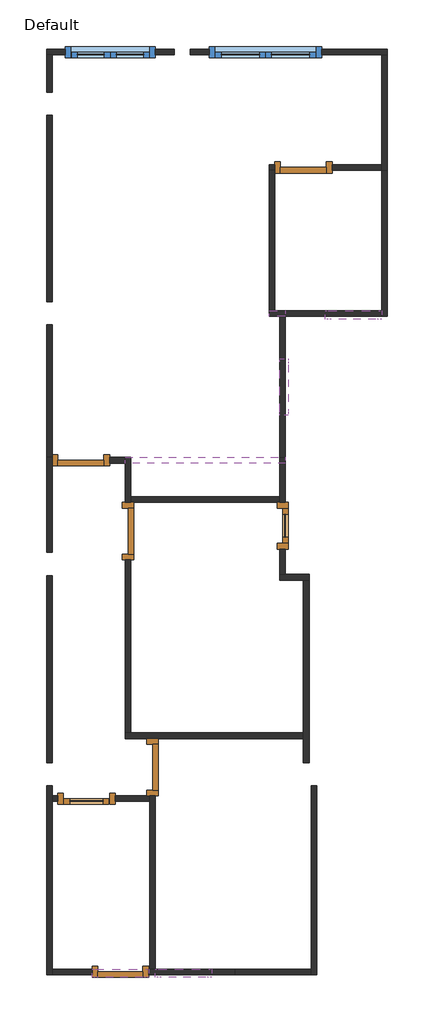
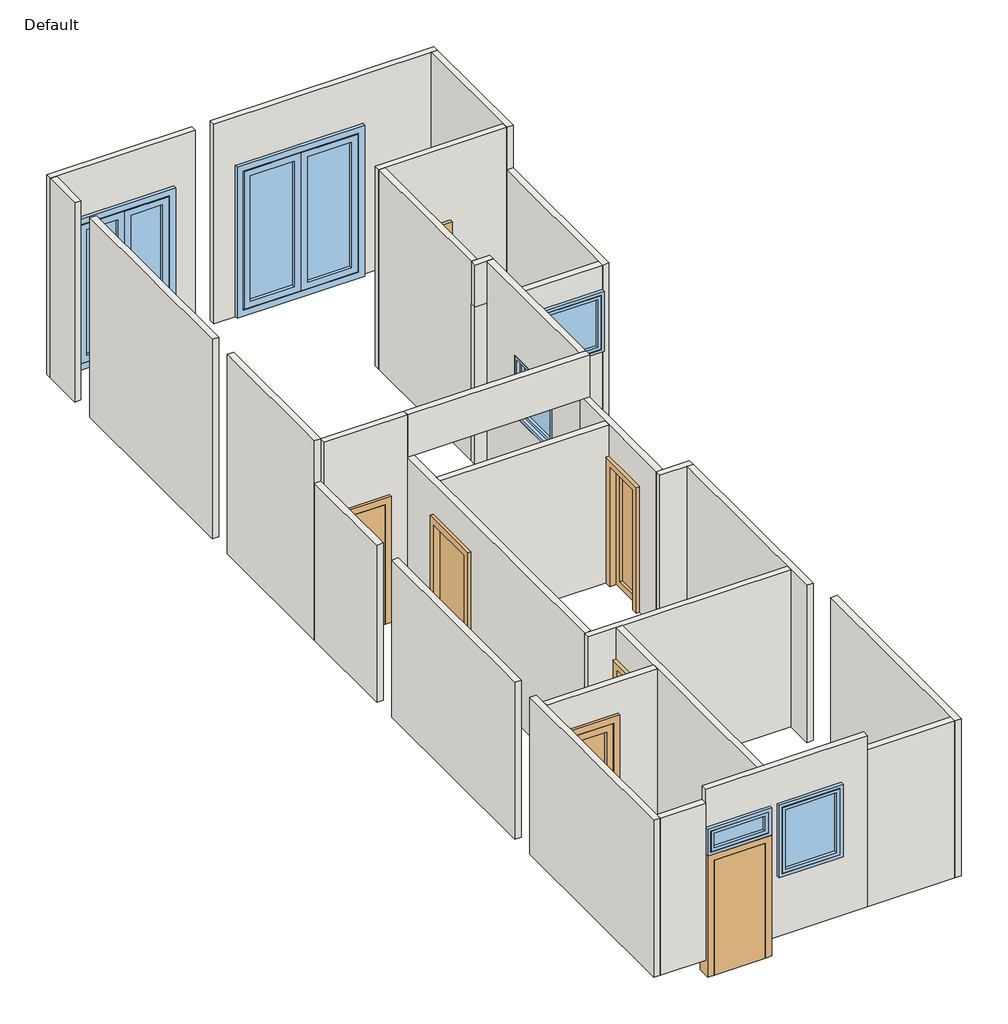
# One storey: 29 walls, 7 doors, 6 windows.
"""IFC4 building model written with IfcOpenShell, lengths in millimetres."""

import ifcopenshell
import ifcopenshell.guid

model = None  # the IFC model being written
_history = None  # IfcOwnerHistory: only IFC2X3 demands one
_inside = {}  # id of a spatial element -> (the spatial element, [elements in it])
_under = {}  # id of a project, library or spatial element -> (it, [spatial elements below it])
_declared = {}  # id of a project -> (the project, [libraries it declares])
_typed = {}  # id of a type object -> (the type object, [elements of that type])
_made_of = {}  # id of a material, layer set ... -> (it, [elements and type objects made of it])


def new_model(schema):
    """Start an empty IFC model of exactly this schema.

    Asked for "IFC4X3", IfcOpenShell would pick the latest addendum, in which some entities
    have other attributes; the version numbers below select the first issue.
    IFC2X3 requires an IfcOwnerHistory on every rooted entity: one is made here for all.
    """
    global model, _history
    if schema == "IFC4X3":
        model = ifcopenshell.file(schema_version=(4, 3, 0, 0))
    else:
        model = ifcopenshell.file(schema=schema)
    _inside.clear()
    _under.clear()
    _declared.clear()
    _typed.clear()
    _made_of.clear()
    _history = None
    if model.schema == "IFC2X3":
        org = make("IfcOrganization", Name="unknown")
        user = make(
            "IfcPersonAndOrganization",
            ThePerson=make("IfcPerson", FamilyName="unknown"),
            TheOrganization=org,
        )
        app = make(
            "IfcApplication",
            ApplicationDeveloper=org,
            Version="unknown",
            ApplicationFullName="unknown",
            ApplicationIdentifier="unknown",
        )
        _history = make(
            "IfcOwnerHistory",
            OwningUser=user,
            OwningApplication=app,
            ChangeAction="ADDED",
            CreationDate=0,
        )
    return model


def make(cls, **values):
    """One entity of the class cls with the attributes given. An attribute that is None is left unset."""
    return model.create_entity(
        cls, **{name: value for name, value in values.items() if value is not None}
    )


def rooted(cls, **values):
    """An entity with a GlobalId (a new one), such as an element, a storey or a relation."""
    return make(cls, GlobalId=ifcopenshell.guid.new(), OwnerHistory=_history, **values)


def si_unit(unit_type, name, prefix=None):
    """IfcSIUnit, for example si_unit("LENGTHUNIT", "METRE", prefix="MILLI")."""
    return make("IfcSIUnit", UnitType=unit_type, Prefix=prefix, Name=name)


def assignment(units):
    """IfcUnitAssignment: the units of a project."""
    return None if units is None else make("IfcUnitAssignment", Units=units)


def point(xyz):
    """IfcCartesianPoint."""
    return None if xyz is None else make("IfcCartesianPoint", Coordinates=xyz)


def direction(xyz):
    """IfcDirection."""
    return None if xyz is None else make("IfcDirection", DirectionRatios=xyz)


def frame(location, z_axis=None, x_axis=None):
    """IfcAxis2Placement3D, a coordinate frame: its origin and axes. An axis left out is left unset."""
    return make(
        "IfcAxis2Placement3D",
        Location=point(location),
        Axis=direction(z_axis),
        RefDirection=direction(x_axis),
    )


def origin():
    """The frame at (0, 0, 0) with its axes left unset."""
    return frame((0.0, 0.0, 0.0))


def origin_with_axes():
    """The frame at (0, 0, 0) with the z axis (0, 0, 1) and the x axis (1, 0, 0) written out."""
    return frame((0.0, 0.0, 0.0), z_axis=(0.0, 0.0, 1.0), x_axis=(1.0, 0.0, 0.0))


def place(relative_to, where):
    """IfcLocalPlacement: puts the frame where relative to a parent placement (None: the world)."""
    return make(
        "IfcLocalPlacement", PlacementRelTo=relative_to, RelativePlacement=where
    )


def context(
    kind, dimensions, precision=None, world=None, true_north=None, identifier=None
):
    """IfcGeometricRepresentationContext, for example the 3D "Model" context."""
    return make(
        "IfcGeometricRepresentationContext",
        ContextIdentifier=identifier,
        ContextType=kind,
        CoordinateSpaceDimension=dimensions,
        Precision=precision,
        WorldCoordinateSystem=world,
        TrueNorth=true_north,
    )


def project(units=None, contexts=None):
    """IfcProject with its units and contexts."""
    return rooted(
        "IfcProject",
        Name="project",
        RepresentationContexts=contexts,
        UnitsInContext=assignment(units),
    )


def spatial(cls, under=None, at=None, **own):
    """A site, building, storey or space (cls), placed at a placement, below another one or the project."""
    s = rooted(cls, ObjectPlacement=at, **own)
    if under is not None:
        _under.setdefault(under.id(), (under, []))[1].append(s)
    return s


def polyline(points):
    """IfcPolyline through the points."""
    return make("IfcPolyline", Points=[point(p) for p in points])


def outline(outer, holes=None, kind="AREA"):
    """IfcArbitraryClosedProfileDef: a profile drawn as a closed curve; with holes, ...WithVoids."""
    if holes is None:
        return make("IfcArbitraryClosedProfileDef", ProfileType=kind, OuterCurve=outer)
    return make(
        "IfcArbitraryProfileDefWithVoids",
        ProfileType=kind,
        OuterCurve=outer,
        InnerCurves=holes,
    )


def extrude(swept, where, along, depth):
    """IfcExtrudedAreaSolid: the profile swept, set in the frame where, extruded along a direction by depth."""
    return make(
        "IfcExtrudedAreaSolid",
        SweptArea=swept,
        Position=where,
        ExtrudedDirection=direction(along),
        Depth=depth,
    )


def shape(context_of_items, identifier, shape_type, items):
    """IfcShapeRepresentation: the items that make up one representation, for example the "Body"."""
    return make(
        "IfcShapeRepresentation",
        ContextOfItems=context_of_items,
        RepresentationIdentifier=identifier,
        RepresentationType=shape_type,
        Items=items,
    )


def source(mapping_origin, context_of_items, identifier, shape_type, items):
    """IfcRepresentationMap: a shape defined once, which mapped items show again and again."""
    return make(
        "IfcRepresentationMap",
        MappingOrigin=mapping_origin,
        MappedRepresentation=shape(context_of_items, identifier, shape_type, items),
    )


def transform(
    local_origin,
    x_axis=None,
    y_axis=None,
    z_axis=None,
    scale=None,
    scale2=None,
    scale3=None,
    uniform=True,
):
    """IfcCartesianTransformationOperator3D, or its non-uniform kind. x_axis, y_axis, z_axis: its Axis1, 2, 3."""
    if uniform:
        return make(
            "IfcCartesianTransformationOperator3D",
            Axis1=direction(x_axis),
            Axis2=direction(y_axis),
            LocalOrigin=point(local_origin),
            Scale=scale,
            Axis3=direction(z_axis),
        )
    return make(
        "IfcCartesianTransformationOperator3DnonUniform",
        Axis1=direction(x_axis),
        Axis2=direction(y_axis),
        LocalOrigin=point(local_origin),
        Scale=scale,
        Axis3=direction(z_axis),
        Scale2=scale2,
        Scale3=scale3,
    )


def mapped(mapping_source, mapping_target):
    """IfcMappedItem: shows the shape of a source again, moved by a transform."""
    return make(
        "IfcMappedItem", MappingSource=mapping_source, MappingTarget=mapping_target
    )


def made_of(thing, what):
    """Note that an element or type object is made of a material, layer set ...; save() writes the relation."""
    if what is not None:
        _made_of.setdefault(what.id(), (what, []))[1].append(thing)
    return thing


def element(
    cls,
    number,
    at=None,
    inside=None,
    cuts=None,
    type_object=None,
    material=None,
    context=None,
    identifier="Body",
    shape_type=None,
    held_by="IfcProductDefinitionShape",
    body=None,
    shapes=None,
    **own,
):
    """One element of the class cls, such as IfcWall. Its Tag is "e" and its number.

    at: its placement. inside: the storey or other place that contains it. cuts: it is an
    opening in that element (IfcRelVoidsElement). A single representation is given by context,
    identifier, shape_type and body (its items); several are given by shapes. held_by: the class
    of the entity that holds the representations. save() writes the other relations.
    """
    e = rooted(cls, Tag="e%d" % number, ObjectPlacement=at, **own)
    if body is not None:
        shapes = [shape(context, identifier, shape_type, body)]
    if shapes is not None:
        e.Representation = make(held_by, Representations=shapes)
    if inside is not None:
        _inside.setdefault(inside.id(), (inside, []))[1].append(e)
    if cuts is not None:
        rooted(
            "IfcRelVoidsElement", RelatingBuildingElement=cuts, RelatedOpeningElement=e
        )
    if type_object is not None:
        _typed.setdefault(type_object.id(), (type_object, []))[1].append(e)
    return made_of(e, material)


def aggregate(whole, parts):
    """IfcRelAggregates: a whole, such as a stair, and the parts it consists of."""
    return rooted("IfcRelAggregates", RelatingObject=whole, RelatedObjects=parts)


def save(model, path):
    """Write the relations noted so far, then the file.

    IfcRelAggregates (storeys below a building ...), IfcRelContainedInSpatialStructure (elements
    in a storey), IfcRelDefinesByType, IfcRelAssociatesMaterial and IfcRelDeclares: one each for
    every whole, place, type object, material and project.
    """
    for whole, parts in _under.values():
        aggregate(whole, parts)
    for where, things in _inside.values():
        rooted(
            "IfcRelContainedInSpatialStructure",
            RelatedElements=things,
            RelatingStructure=where,
        )
    for kind, things in _typed.values():
        rooted("IfcRelDefinesByType", RelatedObjects=things, RelatingType=kind)
    for what, things in _made_of.values():
        rooted("IfcRelAssociatesMaterial", RelatedObjects=things, RelatingMaterial=what)
    for by, libraries in _declared.values():
        rooted("IfcRelDeclares", RelatingContext=by, RelatedDefinitions=libraries)
    model.write(path)


def bathroom_door_bathroom_door_15b6a89a(model_context):
    return source(origin(), model_context, "Body", "SweptSolid", [
        extrude(outline(polyline([(4275.0, 14755.0), (5095.0, 14755.0), (5095.0, 14655.0), (4275.0, 14655.0), (4275.0, 14755.0)])), frame((0.0, 0.0, 250.0), z_axis=(0.0, 0.0, 1.0), x_axis=(1.0, 0.0, 0.0)), (0.0, 0.0, 1.0), 1980.0),
        extrude(outline(polyline([(250.0, 4175.0), (250.0, 4275.0), (2230.0, 4275.0), (2230.0, 5095.0), (250.0, 5095.0), (250.0, 5195.0), (2330.0, 5195.0), (2330.0, 4175.0), (250.0, 4175.0)])), frame((0.0, 14655.0, 0.0), z_axis=(0.0, 1.0, 0.0), x_axis=(0.0, 0.0, 1.0)), (0.0, 0.0, 1.0), 200.0),
    ])


def bedroom_1_door_bedroom_1_door_f4a16035(model_context):
    return source(origin(), model_context, "Body", "SweptSolid", [
        extrude(outline(polyline([(2000.0, 3675.0), (2000.0, 4495.0), (2100.0, 4495.0), (2100.0, 3675.0), (2000.0, 3675.0)])), frame((0.0, 0.0, 250.0), z_axis=(0.0, 0.0, 1.0), x_axis=(1.0, 0.0, 0.0)), (0.0, 0.0, 1.0), 1980.0),
        extrude(outline(polyline([(4595.0, 250.0), (4495.0, 250.0), (4495.0, 2230.0), (3675.0, 2230.0), (3675.0, 250.0), (3575.0, 250.0), (3575.0, 2330.0), (4595.0, 2330.0), (4595.0, 250.0)])), frame((1900.0, 0.0, 0.0), z_axis=(1.0, 0.0, 0.0), x_axis=(0.0, 1.0, 0.0)), (0.0, 0.0, 1.0), 200.0),
    ])


def bedroom_2_door_bedroom_2_door_3f2e3542(model_context):
    return source(origin(), model_context, "Body", "SweptSolid", [
        extrude(outline(polyline([(1565.0, 7875.0), (1565.0, 8695.0), (1665.0, 8695.0), (1665.0, 7875.0), (1565.0, 7875.0)])), frame((0.0, 0.0, 250.0), z_axis=(0.0, 0.0, 1.0), x_axis=(1.0, 0.0, 0.0)), (0.0, 0.0, 1.0), 1980.0),
        extrude(outline(polyline([(8795.0, 250.0), (8695.0, 250.0), (8695.0, 2230.0), (7875.0, 2230.0), (7875.0, 250.0), (7775.0, 250.0), (7775.0, 2330.0), (8795.0, 2330.0), (8795.0, 250.0)])), frame((1465.0, 0.0, 0.0), z_axis=(1.0, 0.0, 0.0), x_axis=(0.0, 1.0, 0.0)), (0.0, 0.0, 1.0), 200.0),
    ])


def bedroom_2_glass_door_bedroom_2_glass_door_faeb561c(model_context):
    return source(origin(), model_context, "Body", "SweptSolid", [
        extrude(outline(polyline([(4355.0, 8175.0), (4355.0, 8585.0), (4365.0, 8585.0), (4365.0, 8175.0), (4355.0, 8175.0)])), frame((0.0, 0.0, 360.0), z_axis=(0.0, 0.0, 1.0), x_axis=(1.0, 0.0, 0.0)), (0.0, 0.0, 1.0), 1760.0),
        extrude(outline(polyline([(8685.0, 2220.0), (8685.0, 260.0), (8075.0, 260.0), (8075.0, 2220.0), (8685.0, 2220.0)]), holes=[polyline([(8585.0, 360.0), (8585.0, 2120.0), (8175.0, 2120.0), (8175.0, 360.0), (8585.0, 360.0)])]), frame((4315.0, 0.0, 0.0), z_axis=(1.0, 0.0, 0.0), x_axis=(0.0, 1.0, 0.0)), (0.0, 0.0, 1.0), 100.0),
        extrude(outline(polyline([(8795.0, 250.0), (8695.0, 250.0), (8695.0, 2230.0), (8065.0, 2230.0), (8065.0, 250.0), (7965.0, 250.0), (7965.0, 2330.0), (8795.0, 2330.0), (8795.0, 250.0)])), frame((4215.0, 0.0, 0.0), z_axis=(1.0, 0.0, 0.0), x_axis=(0.0, 1.0, 0.0)), (0.0, 0.0, 1.0), 200.0),
    ])


def corridor_door_corridor_door_22811d5d(model_context):
    return source(origin(), model_context, "Body", "SweptSolid", [
        extrude(outline(polyline([(525.0, 3485.0), (1125.0, 3485.0), (1125.0, 3475.0), (525.0, 3475.0), (525.0, 3485.0)])), frame((0.0, 0.0, 360.0), z_axis=(0.0, 0.0, 1.0), x_axis=(1.0, 0.0, 0.0)), (0.0, 0.0, 1.0), 1760.0),
        extrude(outline(polyline([(260.0, 1225.0), (2220.0, 1225.0), (2220.0, 425.0), (260.0, 425.0), (260.0, 1225.0)]), holes=[polyline([(360.0, 525.0), (2120.0, 525.0), (2120.0, 1125.0), (360.0, 1125.0), (360.0, 525.0)])]), frame((0.0, 3425.0, 0.0), z_axis=(0.0, 1.0, 0.0), x_axis=(0.0, 0.0, 1.0)), (0.0, 0.0, 1.0), 100.0),
        extrude(outline(polyline([(250.0, 315.0), (250.0, 415.0), (2230.0, 415.0), (2230.0, 1235.0), (250.0, 1235.0), (250.0, 1335.0), (2330.0, 1335.0), (2330.0, 315.0), (250.0, 315.0)])), frame((0.0, 3425.0, 0.0), z_axis=(0.0, 1.0, 0.0), x_axis=(0.0, 0.0, 1.0)), (0.0, 0.0, 1.0), 200.0),
    ])


def front_door_front_door_f10339a7(model_context):
    return source(origin(), model_context, "Body", "SweptSolid", [
        extrude(outline(polyline([(1030.0, 445.0), (1830.0, 445.0), (1830.0, 345.0), (1030.0, 345.0), (1030.0, 445.0)])), origin_with_axes(), (0.0, 0.0, 1.0), 1900.0),
        extrude(outline(polyline([(0.0, 930.0), (0.0, 1030.0), (1900.0, 1030.0), (1900.0, 1830.0), (0.0, 1830.0), (0.0, 1930.0), (2000.0, 1930.0), (2000.0, 930.0), (0.0, 930.0)])), frame((0.0, 345.0, 0.0), z_axis=(0.0, 1.0, 0.0), x_axis=(0.0, 0.0, 1.0)), (0.0, 0.0, 1.0), 200.0),
    ])


def living_room_door_living_room_door_3c1abd9c(model_context):
    return source(origin(), model_context, "Body", "SweptSolid", [
        extrude(outline(polyline([(315.0, 9545.0), (1135.0, 9545.0), (1135.0, 9445.0), (315.0, 9445.0), (315.0, 9545.0)])), frame((0.0, 0.0, 250.0), z_axis=(0.0, 0.0, 1.0), x_axis=(1.0, 0.0, 0.0)), (0.0, 0.0, 1.0), 1980.0),
        extrude(outline(polyline([(250.0, 215.0), (250.0, 315.0), (2230.0, 315.0), (2230.0, 1135.0), (250.0, 1135.0), (250.0, 1235.0), (2330.0, 1235.0), (2330.0, 215.0), (250.0, 215.0)])), frame((0.0, 9445.0, 0.0), z_axis=(0.0, 1.0, 0.0), x_axis=(0.0, 0.0, 1.0)), (0.0, 0.0, 1.0), 200.0),
    ])


def steel_wall_1_steel_wall_1_b92ec2ca(model_context):
    return source(origin(), model_context, "Body", "SweptSolid", [
        extrude(outline(polyline([(215.0, 3755.0), (215.0, 395.0), (115.0, 395.0), (115.0, 3755.0), (215.0, 3755.0)])), frame((0.0, 0.0, 250.0), z_axis=(0.0, 0.0, 1.0), x_axis=(1.0, 0.0, 0.0)), (0.0, 0.0, 1.0), 2600.0),
    ])


def steel_wall_10_1_steel_wall_10_1_b84ba1d7(model_context):
    return source(origin(), model_context, "Body", "SweptSolid", [
        extrude(outline(polyline([(9595.0, 3550.0), (12105.0, 3550.0), (12105.0, 250.0), (9595.0, 250.0), (9595.0, 3550.0)]), holes=[polyline([(11350.0, 2450.0), (10350.0, 2450.0), (10350.0, 1450.0), (11350.0, 1450.0), (11350.0, 2450.0)])]), frame((4265.0, 0.0, 0.0), z_axis=(1.0, 0.0, 0.0), x_axis=(0.0, 1.0, 0.0)), (0.0, 0.0, 1.0), 100.0),
    ])


def steel_wall_10_2_steel_wall_10_2_ac5a625b(model_context):
    return source(origin(), model_context, "Body", "SweptSolid", [
        extrude(outline(polyline([(7515.0, 2850.0), (9595.0, 2850.0), (9595.0, 250.0), (8795.0, 250.0), (8795.0, 2330.0), (7965.0, 2330.0), (7965.0, 250.0), (7515.0, 250.0), (7515.0, 2850.0)])), frame((4265.0, 0.0, 0.0), z_axis=(1.0, 0.0, 0.0), x_axis=(0.0, 1.0, 0.0)), (0.0, 0.0, 1.0), 100.0),
    ])


def steel_wall_11_steel_wall_11_b2c771ff(model_context):
    return source(origin(), model_context, "Body", "SweptSolid", [
        extrude(outline(polyline([(4785.0, 7415.0), (4265.0, 7415.0), (4265.0, 7515.0), (4785.0, 7515.0), (4785.0, 7415.0)])), frame((0.0, 0.0, 250.0), z_axis=(0.0, 0.0, 1.0), x_axis=(1.0, 0.0, 0.0)), (0.0, 0.0, 1.0), 2600.0),
    ])


def steel_wall_12_steel_wall_12_e47ad89f(model_context):
    return source(origin(), model_context, "Body", "SweptSolid", [
        extrude(outline(polyline([(4785.0, 7415.0), (4785.0, 4165.0), (4685.0, 4165.0), (4685.0, 7415.0), (4785.0, 7415.0)])), frame((0.0, 0.0, 250.0), z_axis=(0.0, 0.0, 1.0), x_axis=(1.0, 0.0, 0.0)), (0.0, 0.0, 1.0), 2600.0),
    ])


def steel_wall_13_steel_wall_13_94e184f7(model_context):
    return source(origin(), model_context, "Body", "SweptSolid", [
        extrude(outline(polyline([(4925.0, 3755.0), (4925.0, 395.0), (4825.0, 395.0), (4825.0, 3755.0), (4925.0, 3755.0)])), frame((0.0, 0.0, 250.0), z_axis=(0.0, 0.0, 1.0), x_axis=(1.0, 0.0, 0.0)), (0.0, 0.0, 1.0), 2600.0),
    ])


def steel_wall_14_1_steel_wall_14_1_bad66547(model_context):
    return source(origin(), model_context, "Body", "SweptSolid", [
        extrude(outline(polyline([(930.0, 395.0), (215.0, 395.0), (215.0, 495.0), (930.0, 495.0), (930.0, 395.0)])), frame((0.0, 0.0, 250.0), z_axis=(0.0, 0.0, 1.0), x_axis=(1.0, 0.0, 0.0)), (0.0, 0.0, 1.0), 2600.0),
    ])


def steel_wall_14_2_steel_wall_14_2_555e5885(model_context):
    return source(origin(), model_context, "Body", "SweptSolid", [
        extrude(outline(polyline([(3080.0, 3460.0), (3080.0, 930.0), (2450.0, 930.0), (2450.0, 1930.0), (250.0, 1930.0), (250.0, 3460.0), (3080.0, 3460.0)]), holes=[polyline([(2450.0, 2050.0), (2450.0, 3050.0), (1250.0, 3050.0), (1250.0, 2050.0), (2450.0, 2050.0)])]), frame((0.0, 395.0, 0.0), z_axis=(0.0, 1.0, 0.0), x_axis=(0.0, 0.0, 1.0)), (0.0, 0.0, 1.0), 100.0),
    ])


def steel_wall_14_3_steel_wall_14_3_bb8a6b82(model_context):
    return source(origin(), model_context, "Body", "SweptSolid", [
        extrude(outline(polyline([(4825.0, 395.0), (3460.0, 395.0), (3460.0, 495.0), (4825.0, 495.0), (4825.0, 395.0)])), frame((0.0, 0.0, 250.0), z_axis=(0.0, 0.0, 1.0), x_axis=(1.0, 0.0, 0.0)), (0.0, 0.0, 1.0), 2600.0),
    ])


def steel_wall_2_steel_wall_2_9d9e34b6(model_context):
    return source(origin(), model_context, "Body", "SweptSolid", [
        extrude(outline(polyline([(215.0, 7495.0), (215.0, 4165.0), (115.0, 4165.0), (115.0, 7495.0), (215.0, 7495.0)])), frame((0.0, 0.0, 250.0), z_axis=(0.0, 0.0, 1.0), x_axis=(1.0, 0.0, 0.0)), (0.0, 0.0, 1.0), 2600.0),
    ])


def steel_wall_3_1_steel_wall_3_1_bd8174d4(model_context):
    return source(origin(), model_context, "Body", "SweptSolid", [
        extrude(outline(polyline([(215.0, 9595.0), (215.0, 7905.0), (115.0, 7905.0), (115.0, 9595.0), (215.0, 9595.0)])), frame((0.0, 0.0, 250.0), z_axis=(0.0, 0.0, 1.0), x_axis=(1.0, 0.0, 0.0)), (0.0, 0.0, 1.0), 2600.0),
    ])


def steel_wall_3_2_steel_wall_3_2_60cdce26(model_context):
    return source(origin(), model_context, "Body", "SweptSolid", [
        extrude(outline(polyline([(215.0, 11955.0), (215.0, 9595.0), (115.0, 9595.0), (115.0, 11955.0), (215.0, 11955.0)])), frame((0.0, 0.0, 250.0), z_axis=(0.0, 0.0, 1.0), x_axis=(1.0, 0.0, 0.0)), (0.0, 0.0, 1.0), 3300.0),
    ])


def steel_wall_4_steel_wall_4_2983a264(model_context):
    return source(origin(), model_context, "Body", "SweptSolid", [
        extrude(outline(polyline([(215.0, 15685.0), (215.0, 12365.0), (115.0, 12365.0), (115.0, 15685.0), (215.0, 15685.0)])), frame((0.0, 0.0, 250.0), z_axis=(0.0, 0.0, 1.0), x_axis=(1.0, 0.0, 0.0)), (0.0, 0.0, 1.0), 3300.0),
    ])


def steel_wall_5_steel_wall_5_69cba077(model_context):
    return source(origin(), model_context, "Body", "SweptSolid", [
        extrude(outline(polyline([(215.0, 16755.0), (215.0, 16095.0), (115.0, 16095.0), (115.0, 16755.0), (215.0, 16755.0)])), frame((0.0, 0.0, 250.0), z_axis=(0.0, 0.0, 1.0), x_axis=(1.0, 0.0, 0.0)), (0.0, 0.0, 1.0), 3300.0),
    ])


def steel_wall_6_steel_wall_6_a34f8d7e(model_context):
    return source(origin(), model_context, "Body", "SweptSolid", [
        extrude(outline(polyline([(3550.0, 2385.0), (3550.0, 115.0), (250.0, 115.0), (250.0, 450.0), (2750.0, 450.0), (2750.0, 2050.0), (250.0, 2050.0), (250.0, 2385.0), (3550.0, 2385.0)])), frame((0.0, 16755.0, 0.0), z_axis=(0.0, 1.0, 0.0), x_axis=(0.0, 0.0, 1.0)), (0.0, 0.0, 1.0), 100.0),
    ])


def steel_wall_7_steel_wall_7_8661bafb(model_context):
    return source(origin(), model_context, "Body", "SweptSolid", [
        extrude(outline(polyline([(3550.0, 6175.0), (3550.0, 2675.0), (250.0, 2675.0), (250.0, 3010.0), (2750.0, 3010.0), (2750.0, 5010.0), (250.0, 5010.0), (250.0, 6175.0), (3550.0, 6175.0)])), frame((0.0, 16755.0, 0.0), z_axis=(0.0, 1.0, 0.0), x_axis=(0.0, 0.0, 1.0)), (0.0, 0.0, 1.0), 100.0),
    ])


def steel_wall_8_1_steel_wall_8_1_6002a07f(model_context):
    return source(origin(), model_context, "Body", "SweptSolid", [
        extrude(outline(polyline([(6175.0, 16755.0), (6175.0, 14705.0), (6075.0, 14705.0), (6075.0, 16755.0), (6175.0, 16755.0)])), frame((0.0, 0.0, 250.0), z_axis=(0.0, 0.0, 1.0), x_axis=(1.0, 0.0, 0.0)), (0.0, 0.0, 1.0), 3300.0),
    ])


def steel_wall_8_2_steel_wall_8_2_e95248a5(model_context):
    return source(origin(), model_context, "Body", "SweptSolid", [
        extrude(outline(polyline([(6175.0, 14705.0), (6175.0, 12105.0), (6075.0, 12105.0), (6075.0, 14705.0), (6175.0, 14705.0)])), frame((0.0, 0.0, 250.0), z_axis=(0.0, 0.0, 1.0), x_axis=(1.0, 0.0, 0.0)), (0.0, 0.0, 1.0), 2600.0),
    ])


def steel_wall_9_steel_wall_9_7bb1e214(model_context):
    return source(origin(), model_context, "Body", "SweptSolid", [
        extrude(outline(polyline([(2850.0, 6075.0), (2850.0, 4075.0), (250.0, 4075.0), (250.0, 6075.0), (1450.0, 6075.0), (1450.0, 5075.0), (2450.0, 5075.0), (2450.0, 6075.0), (2850.0, 6075.0)])), frame((0.0, 12105.0, 0.0), z_axis=(0.0, 1.0, 0.0), x_axis=(0.0, 0.0, 1.0)), (0.0, 0.0, 1.0), 100.0),
    ])


def steel_wall_bath_1_steel_wall_bath_1_50d80b11(model_context):
    return source(origin(), model_context, "Body", "SweptSolid", [
        extrude(outline(polyline([(4175.0, 14705.0), (4175.0, 12205.0), (4075.0, 12205.0), (4075.0, 14705.0), (4175.0, 14705.0)])), frame((0.0, 0.0, 250.0), z_axis=(0.0, 0.0, 1.0), x_axis=(1.0, 0.0, 0.0)), (0.0, 0.0, 1.0), 3300.0),
    ])


def steel_wall_bath_2_steel_wall_bath_2_118e7a6d(model_context):
    return source(origin(), model_context, "Body", "SweptSolid", [
        extrude(outline(polyline([(3550.0, 6075.0), (3550.0, 4075.0), (250.0, 4075.0), (250.0, 4175.0), (2330.0, 4175.0), (2330.0, 5195.0), (250.0, 5195.0), (250.0, 6075.0), (3550.0, 6075.0)])), frame((0.0, 14705.0, 0.0), z_axis=(0.0, 1.0, 0.0), x_axis=(0.0, 0.0, 1.0)), (0.0, 0.0, 1.0), 100.0),
    ])


def steel_wall_bath_3_steel_wall_bath_3_592d521f(model_context):
    return source(origin(), model_context, "Body", "SweptSolid", [
        extrude(outline(polyline([(4365.0, 12105.0), (4075.0, 12105.0), (4075.0, 12205.0), (4365.0, 12205.0), (4365.0, 12105.0)])), frame((0.0, 0.0, 2850.0), z_axis=(0.0, 0.0, 1.0), x_axis=(1.0, 0.0, 0.0)), (0.0, 0.0, 1.0), 700.0),
    ])


def steel_wall_bed_1_1_steel_wall_bed_1_1_07c56df4(model_context):
    return source(origin(), model_context, "Body", "SweptSolid", [
        extrude(outline(polyline([(495.0, 2850.0), (4595.0, 2850.0), (4595.0, 2330.0), (3575.0, 2330.0), (3575.0, 250.0), (495.0, 250.0), (495.0, 2850.0)])), frame((1950.0, 0.0, 0.0), z_axis=(1.0, 0.0, 0.0), x_axis=(0.0, 1.0, 0.0)), (0.0, 0.0, 1.0), 100.0),
    ])


def steel_wall_bed_1_2_steel_wall_bed_1_2_5afbed24(model_context):
    return source(origin(), model_context, "Body", "SweptSolid", [
        extrude(outline(polyline([(4685.0, 4595.0), (1515.0, 4595.0), (1515.0, 4695.0), (4685.0, 4695.0), (4685.0, 4595.0)])), frame((0.0, 0.0, 250.0), z_axis=(0.0, 0.0, 1.0), x_axis=(1.0, 0.0, 0.0)), (0.0, 0.0, 1.0), 2600.0),
    ])


def steel_wall_bed_2_1_steel_wall_bed_2_1_f0eb02fb(model_context):
    return source(origin(), model_context, "Body", "SweptSolid", [
        extrude(outline(polyline([(4695.0, 2850.0), (9595.0, 2850.0), (9595.0, 250.0), (8795.0, 250.0), (8795.0, 2330.0), (7775.0, 2330.0), (7775.0, 250.0), (4695.0, 250.0), (4695.0, 2850.0)])), frame((1515.0, 0.0, 0.0), z_axis=(1.0, 0.0, 0.0), x_axis=(0.0, 1.0, 0.0)), (0.0, 0.0, 1.0), 100.0),
    ])


def steel_wall_bed_2_2_steel_wall_bed_2_2_f5710ee6(model_context):
    return source(origin(), model_context, "Body", "SweptSolid", [
        extrude(outline(polyline([(4265.0, 8795.0), (1615.0, 8795.0), (1615.0, 8895.0), (4265.0, 8895.0), (4265.0, 8795.0)])), frame((0.0, 0.0, 250.0), z_axis=(0.0, 0.0, 1.0), x_axis=(1.0, 0.0, 0.0)), (0.0, 0.0, 1.0), 2600.0),
    ])


def steel_wall_corridor_1_steel_wall_corridor_1_64942479(model_context):
    return source(origin(), model_context, "Body", "SweptSolid", [
        extrude(outline(polyline([(2850.0, 1950.0), (2850.0, 215.0), (250.0, 215.0), (250.0, 315.0), (2330.0, 315.0), (2330.0, 1335.0), (250.0, 1335.0), (250.0, 1950.0), (2850.0, 1950.0)])), frame((0.0, 3475.0, 0.0), z_axis=(0.0, 1.0, 0.0), x_axis=(0.0, 0.0, 1.0)), (0.0, 0.0, 1.0), 100.0),
    ])


def steel_wall_corridor_2_steel_wall_corridor_2_3c3fb1a4(model_context):
    return source(origin(), model_context, "Body", "SweptSolid", [
        extrude(outline(polyline([(3550.0, 1515.0), (3550.0, 215.0), (2330.0, 215.0), (2330.0, 1235.0), (250.0, 1235.0), (250.0, 1515.0), (3550.0, 1515.0)])), frame((0.0, 9495.0, 0.0), z_axis=(0.0, 1.0, 0.0), x_axis=(0.0, 0.0, 1.0)), (0.0, 0.0, 1.0), 100.0),
    ])


def steel_wall_kitchen_steel_wall_kitchen_7f8e7296(model_context):
    return source(origin(), model_context, "Body", "SweptSolid", [
        extrude(outline(polyline([(4365.0, 9495.0), (1515.0, 9495.0), (1515.0, 9595.0), (4365.0, 9595.0), (4365.0, 9495.0)])), frame((0.0, 0.0, 2850.0), z_axis=(0.0, 0.0, 1.0), x_axis=(1.0, 0.0, 0.0)), (0.0, 0.0, 1.0), 700.0),
    ])


def bedroom_1_window_bedroom_1_window_a7b937d5(model_context):
    return source(origin(), model_context, "Body", "SweptSolid", [
        extrude(outline(polyline([(5180.0, 12115.0), (5970.0, 12115.0), (5970.0, 12105.0), (5180.0, 12105.0), (5180.0, 12115.0)])), frame((0.0, 0.0, 1555.0), z_axis=(0.0, 0.0, 1.0), x_axis=(1.0, 0.0, 0.0)), (0.0, 0.0, 1.0), 790.0),
        extrude(outline(polyline([(1505.0, 6020.0), (2395.0, 6020.0), (2395.0, 5130.0), (1505.0, 5130.0), (1505.0, 6020.0)]), holes=[polyline([(1555.0, 5180.0), (2345.0, 5180.0), (2345.0, 5970.0), (1555.0, 5970.0), (1555.0, 5180.0)])]), frame((0.0, 12055.0, 0.0), z_axis=(0.0, 1.0, 0.0), x_axis=(0.0, 0.0, 1.0)), (0.0, 0.0, 1.0), 100.0),
        extrude(outline(polyline([(1450.0, 6075.0), (2450.0, 6075.0), (2450.0, 5075.0), (1450.0, 5075.0), (1450.0, 6075.0)]), holes=[polyline([(1500.0, 5125.0), (2400.0, 5125.0), (2400.0, 6025.0), (1500.0, 6025.0), (1500.0, 5125.0)])]), frame((0.0, 12055.0, 0.0), z_axis=(0.0, 1.0, 0.0), x_axis=(0.0, 0.0, 1.0)), (0.0, 0.0, 1.0), 150.0),
    ])


def bedroom_1_window001_bedroom_1_window001_719b1152(model_context):
    return source(origin(), model_context, "Body", "SweptSolid", [
        extrude(outline(polyline([(2155.0, 405.0), (2945.0, 405.0), (2945.0, 395.0), (2155.0, 395.0), (2155.0, 405.0)])), frame((0.0, 0.0, 1355.0), z_axis=(0.0, 0.0, 1.0), x_axis=(1.0, 0.0, 0.0)), (0.0, 0.0, 1.0), 990.0),
        extrude(outline(polyline([(1305.0, 2995.0), (2395.0, 2995.0), (2395.0, 2105.0), (1305.0, 2105.0), (1305.0, 2995.0)]), holes=[polyline([(1355.0, 2155.0), (2345.0, 2155.0), (2345.0, 2945.0), (1355.0, 2945.0), (1355.0, 2155.0)])]), frame((0.0, 345.0, 0.0), z_axis=(0.0, 1.0, 0.0), x_axis=(0.0, 0.0, 1.0)), (0.0, 0.0, 1.0), 100.0),
        extrude(outline(polyline([(1250.0, 3050.0), (2450.0, 3050.0), (2450.0, 2050.0), (1250.0, 2050.0), (1250.0, 3050.0)]), holes=[polyline([(1300.0, 2100.0), (2400.0, 2100.0), (2400.0, 3000.0), (1300.0, 3000.0), (1300.0, 2100.0)])]), frame((0.0, 345.0, 0.0), z_axis=(0.0, 1.0, 0.0), x_axis=(0.0, 0.0, 1.0)), (0.0, 0.0, 1.0), 150.0),
    ])


def corridor_window_corridor_window_b9059d84(model_context):
    return source(origin(), model_context, "Body", "SweptSolid", [
        extrude(outline(polyline([(1035.0, 405.0), (1825.0, 405.0), (1825.0, 395.0), (1035.0, 395.0), (1035.0, 405.0)])), frame((0.0, 0.0, 2105.0), z_axis=(0.0, 0.0, 1.0), x_axis=(1.0, 0.0, 0.0)), (0.0, 0.0, 1.0), 240.0),
        extrude(outline(polyline([(2055.0, 1875.0), (2395.0, 1875.0), (2395.0, 985.0), (2055.0, 985.0), (2055.0, 1875.0)]), holes=[polyline([(2105.0, 1035.0), (2345.0, 1035.0), (2345.0, 1825.0), (2105.0, 1825.0), (2105.0, 1035.0)])]), frame((0.0, 345.0, 0.0), z_axis=(0.0, 1.0, 0.0), x_axis=(0.0, 0.0, 1.0)), (0.0, 0.0, 1.0), 100.0),
        extrude(outline(polyline([(2000.0, 1930.0), (2450.0, 1930.0), (2450.0, 930.0), (2000.0, 930.0), (2000.0, 1930.0)]), holes=[polyline([(2050.0, 980.0), (2400.0, 980.0), (2400.0, 1880.0), (2050.0, 1880.0), (2050.0, 980.0)])]), frame((0.0, 345.0, 0.0), z_axis=(0.0, 1.0, 0.0), x_axis=(0.0, 0.0, 1.0)), (0.0, 0.0, 1.0), 150.0),
    ])


def garden_door_1_garden_door_1_5a744e37(model_context):
    return source(origin(), model_context, "Body", "SweptSolid", [
        extrude(outline(polyline([(1355.0, 16765.0), (1840.0, 16765.0), (1840.0, 16755.0), (1355.0, 16755.0), (1355.0, 16765.0)])), frame((0.0, 0.0, 460.0), z_axis=(0.0, 0.0, 1.0), x_axis=(1.0, 0.0, 0.0)), (0.0, 0.0, 1.0), 2080.0),
        extrude(outline(polyline([(360.0, 1940.0), (2640.0, 1940.0), (2640.0, 1255.0), (360.0, 1255.0), (360.0, 1940.0)]), holes=[polyline([(460.0, 1355.0), (2540.0, 1355.0), (2540.0, 1840.0), (460.0, 1840.0), (460.0, 1355.0)])]), frame((0.0, 16705.0, 0.0), z_axis=(0.0, 1.0, 0.0), x_axis=(0.0, 0.0, 1.0)), (0.0, 0.0, 1.0), 100.0),
        extrude(outline(polyline([(660.0, 16765.0), (1145.0, 16765.0), (1145.0, 16755.0), (660.0, 16755.0), (660.0, 16765.0)])), frame((0.0, 0.0, 460.0), z_axis=(0.0, 0.0, 1.0), x_axis=(1.0, 0.0, 0.0)), (0.0, 0.0, 1.0), 2080.0),
        extrude(outline(polyline([(360.0, 1245.0), (2640.0, 1245.0), (2640.0, 560.0), (360.0, 560.0), (360.0, 1245.0)]), holes=[polyline([(460.0, 660.0), (2540.0, 660.0), (2540.0, 1145.0), (460.0, 1145.0), (460.0, 660.0)])]), frame((0.0, 16705.0, 0.0), z_axis=(0.0, 1.0, 0.0), x_axis=(0.0, 0.0, 1.0)), (0.0, 0.0, 1.0), 100.0),
        extrude(outline(polyline([(250.0, 2050.0), (2750.0, 2050.0), (2750.0, 450.0), (250.0, 450.0), (250.0, 2050.0)]), holes=[polyline([(350.0, 550.0), (2650.0, 550.0), (2650.0, 1950.0), (350.0, 1950.0), (350.0, 550.0)])]), frame((0.0, 16705.0, 0.0), z_axis=(0.0, 1.0, 0.0), x_axis=(0.0, 0.0, 1.0)), (0.0, 0.0, 1.0), 200.0),
    ])


def garden_door_2_garden_door_2_d5e40104(model_context):
    return source(origin(), model_context, "Body", "SweptSolid", [
        extrude(outline(polyline([(4115.0, 16765.0), (4800.0, 16765.0), (4800.0, 16755.0), (4115.0, 16755.0), (4115.0, 16765.0)])), frame((0.0, 0.0, 460.0), z_axis=(0.0, 0.0, 1.0), x_axis=(1.0, 0.0, 0.0)), (0.0, 0.0, 1.0), 2080.0),
        extrude(outline(polyline([(360.0, 4900.0), (2640.0, 4900.0), (2640.0, 4015.0), (360.0, 4015.0), (360.0, 4900.0)]), holes=[polyline([(460.0, 4115.0), (2540.0, 4115.0), (2540.0, 4800.0), (460.0, 4800.0), (460.0, 4115.0)])]), frame((0.0, 16705.0, 0.0), z_axis=(0.0, 1.0, 0.0), x_axis=(0.0, 0.0, 1.0)), (0.0, 0.0, 1.0), 100.0),
        extrude(outline(polyline([(3220.0, 16765.0), (3905.0, 16765.0), (3905.0, 16755.0), (3220.0, 16755.0), (3220.0, 16765.0)])), frame((0.0, 0.0, 460.0), z_axis=(0.0, 0.0, 1.0), x_axis=(1.0, 0.0, 0.0)), (0.0, 0.0, 1.0), 2080.0),
        extrude(outline(polyline([(360.0, 4005.0), (2640.0, 4005.0), (2640.0, 3120.0), (360.0, 3120.0), (360.0, 4005.0)]), holes=[polyline([(460.0, 3220.0), (2540.0, 3220.0), (2540.0, 3905.0), (460.0, 3905.0), (460.0, 3220.0)])]), frame((0.0, 16705.0, 0.0), z_axis=(0.0, 1.0, 0.0), x_axis=(0.0, 0.0, 1.0)), (0.0, 0.0, 1.0), 100.0),
        extrude(outline(polyline([(250.0, 5010.0), (2750.0, 5010.0), (2750.0, 3010.0), (250.0, 3010.0), (250.0, 5010.0)]), holes=[polyline([(350.0, 3110.0), (2650.0, 3110.0), (2650.0, 4910.0), (350.0, 4910.0), (350.0, 3110.0)])]), frame((0.0, 16705.0, 0.0), z_axis=(0.0, 1.0, 0.0), x_axis=(0.0, 0.0, 1.0)), (0.0, 0.0, 1.0), 200.0),
    ])


def kitchen_window_kitchen_window_f07ff302(model_context):
    return source(origin(), model_context, "Body", "SweptSolid", [
        extrude(outline(polyline([(4355.0, 10455.0), (4355.0, 11245.0), (4365.0, 11245.0), (4365.0, 10455.0), (4355.0, 10455.0)])), frame((0.0, 0.0, 1555.0), z_axis=(0.0, 0.0, 1.0), x_axis=(1.0, 0.0, 0.0)), (0.0, 0.0, 1.0), 790.0),
        extrude(outline(polyline([(11295.0, 2395.0), (11295.0, 1505.0), (10405.0, 1505.0), (10405.0, 2395.0), (11295.0, 2395.0)]), holes=[polyline([(11245.0, 1555.0), (11245.0, 2345.0), (10455.0, 2345.0), (10455.0, 1555.0), (11245.0, 1555.0)])]), frame((4315.0, 0.0, 0.0), z_axis=(1.0, 0.0, 0.0), x_axis=(0.0, 1.0, 0.0)), (0.0, 0.0, 1.0), 100.0),
        extrude(outline(polyline([(11350.0, 2450.0), (11350.0, 1450.0), (10350.0, 1450.0), (10350.0, 2450.0), (11350.0, 2450.0)]), holes=[polyline([(11300.0, 1500.0), (11300.0, 2400.0), (10400.0, 2400.0), (10400.0, 1500.0), (11300.0, 1500.0)])]), frame((4265.0, 0.0, 0.0), z_axis=(1.0, 0.0, 0.0), x_axis=(0.0, 1.0, 0.0)), (0.0, 0.0, 1.0), 150.0),
    ])


model = new_model("IFC4")

# Units and contexts
model_context = context("Model", 3, world=origin())
ifc_project = project(units=[si_unit("LENGTHUNIT", "METRE", prefix="MILLI")], contexts=[model_context])

# Site, building, storey
site = spatial("IfcSite", under=ifc_project)
building = spatial("IfcBuilding", under=site)
storey = spatial("IfcBuildingStorey", under=building, Name="Default", Elevation=0.0)

# Doors
placement = place(None, origin())
bathroom_door_bathroom_door_shape = bathroom_door_bathroom_door_15b6a89a(model_context)
element("IfcDoor", 1, ObjectType="Bathroom_Door : Bathroom_Door", at=placement, inside=storey, context=model_context, shape_type="MappedRepresentation", body=[
    mapped(bathroom_door_bathroom_door_shape, transform((0.0, 0.0, 0.0), x_axis=(1.0, 0.0, 0.0), y_axis=(0.0, 1.0, 0.0), z_axis=(0.0, 0.0, 1.0))),
])
bedroom_1_door_bedroom_1_door_shape = bedroom_1_door_bedroom_1_door_f4a16035(model_context)
element("IfcDoor", 2, ObjectType="Bedroom_1_Door : Bedroom_1_Door", at=placement, inside=storey, context=model_context, shape_type="MappedRepresentation", body=[
    mapped(bedroom_1_door_bedroom_1_door_shape, transform((0.0, 0.0, 0.0), x_axis=(1.0, 0.0, 0.0), y_axis=(0.0, 1.0, 0.0), z_axis=(0.0, 0.0, 1.0))),
])
bedroom_2_door_bedroom_2_door_shape = bedroom_2_door_bedroom_2_door_3f2e3542(model_context)
element("IfcDoor", 3, ObjectType="Bedroom_2_Door : Bedroom_2_Door", at=placement, inside=storey, context=model_context, shape_type="MappedRepresentation", body=[
    mapped(bedroom_2_door_bedroom_2_door_shape, transform((0.0, 0.0, 0.0), x_axis=(1.0, 0.0, 0.0), y_axis=(0.0, 1.0, 0.0), z_axis=(0.0, 0.0, 1.0))),
])
bedroom_2_glass_door_bedroom_2_glass_door_shape = bedroom_2_glass_door_bedroom_2_glass_door_faeb561c(model_context)
element("IfcDoor", 4, ObjectType="Bedroom_2__Glass_Door : Bedroom_2__Glass_Door", at=placement, inside=storey, context=model_context, shape_type="MappedRepresentation", body=[
    mapped(bedroom_2_glass_door_bedroom_2_glass_door_shape, transform((0.0, 0.0, 0.0), x_axis=(1.0, 0.0, 0.0), y_axis=(0.0, 1.0, 0.0), z_axis=(0.0, 0.0, 1.0))),
])
corridor_door_corridor_door_shape = corridor_door_corridor_door_22811d5d(model_context)
element("IfcDoor", 5, ObjectType="Corridor_Door : Corridor_Door", at=placement, inside=storey, context=model_context, shape_type="MappedRepresentation", body=[
    mapped(corridor_door_corridor_door_shape, transform((0.0, 0.0, 0.0), x_axis=(1.0, 0.0, 0.0), y_axis=(0.0, 1.0, 0.0), z_axis=(0.0, 0.0, 1.0))),
])
front_door_front_door_shape = front_door_front_door_f10339a7(model_context)
element("IfcDoor", 6, ObjectType="Front_Door : Front_Door", at=placement, inside=storey, context=model_context, shape_type="MappedRepresentation", body=[
    mapped(front_door_front_door_shape, transform((0.0, 0.0, 0.0), x_axis=(1.0, 0.0, 0.0), y_axis=(0.0, 1.0, 0.0), z_axis=(0.0, 0.0, 1.0))),
])
living_room_door_living_room_door_shape = living_room_door_living_room_door_3c1abd9c(model_context)
element("IfcDoor", 7, ObjectType="Living_Room_Door : Living_Room_Door", at=placement, inside=storey, context=model_context, shape_type="MappedRepresentation", body=[
    mapped(living_room_door_living_room_door_shape, transform((0.0, 0.0, 0.0), x_axis=(1.0, 0.0, 0.0), y_axis=(0.0, 1.0, 0.0), z_axis=(0.0, 0.0, 1.0))),
])

# Walls
steel_wall_1_steel_wall_1_shape = steel_wall_1_steel_wall_1_b92ec2ca(model_context)
element("IfcWall", 8, ObjectType="Steel_Wall_1 : Steel_Wall_1", at=placement, inside=storey, context=model_context, shape_type="MappedRepresentation", body=[
    mapped(steel_wall_1_steel_wall_1_shape, transform((0.0, 0.0, 0.0), x_axis=(1.0, 0.0, 0.0), y_axis=(0.0, 1.0, 0.0), z_axis=(0.0, 0.0, 1.0))),
])
steel_wall_10_1_steel_wall_10_1_shape = steel_wall_10_1_steel_wall_10_1_b84ba1d7(model_context)
element("IfcWall", 9, ObjectType="Steel_Wall_10_1 : Steel_Wall_10_1", at=placement, inside=storey, context=model_context, shape_type="MappedRepresentation", body=[
    mapped(steel_wall_10_1_steel_wall_10_1_shape, transform((0.0, 0.0, 0.0), x_axis=(1.0, 0.0, 0.0), y_axis=(0.0, 1.0, 0.0), z_axis=(0.0, 0.0, 1.0))),
])
steel_wall_10_2_steel_wall_10_2_shape = steel_wall_10_2_steel_wall_10_2_ac5a625b(model_context)
element("IfcWall", 10, ObjectType="Steel_Wall_10_2 : Steel_Wall_10_2", at=placement, inside=storey, context=model_context, shape_type="MappedRepresentation", body=[
    mapped(steel_wall_10_2_steel_wall_10_2_shape, transform((0.0, 0.0, 0.0), x_axis=(1.0, 0.0, 0.0), y_axis=(0.0, 1.0, 0.0), z_axis=(0.0, 0.0, 1.0))),
])
steel_wall_11_steel_wall_11_shape = steel_wall_11_steel_wall_11_b2c771ff(model_context)
element("IfcWall", 11, ObjectType="Steel_Wall_11 : Steel_Wall_11", at=placement, inside=storey, context=model_context, shape_type="MappedRepresentation", body=[
    mapped(steel_wall_11_steel_wall_11_shape, transform((0.0, 0.0, 0.0), x_axis=(1.0, 0.0, 0.0), y_axis=(0.0, 1.0, 0.0), z_axis=(0.0, 0.0, 1.0))),
])
steel_wall_12_steel_wall_12_shape = steel_wall_12_steel_wall_12_e47ad89f(model_context)
element("IfcWall", 12, ObjectType="Steel_Wall_12 : Steel_Wall_12", at=placement, inside=storey, context=model_context, shape_type="MappedRepresentation", body=[
    mapped(steel_wall_12_steel_wall_12_shape, transform((0.0, 0.0, 0.0), x_axis=(1.0, 0.0, 0.0), y_axis=(0.0, 1.0, 0.0), z_axis=(0.0, 0.0, 1.0))),
])
steel_wall_13_steel_wall_13_shape = steel_wall_13_steel_wall_13_94e184f7(model_context)
element("IfcWall", 13, ObjectType="Steel_Wall_13 : Steel_Wall_13", at=placement, inside=storey, context=model_context, shape_type="MappedRepresentation", body=[
    mapped(steel_wall_13_steel_wall_13_shape, transform((0.0, 0.0, 0.0), x_axis=(1.0, 0.0, 0.0), y_axis=(0.0, 1.0, 0.0), z_axis=(0.0, 0.0, 1.0))),
])
steel_wall_14_1_steel_wall_14_1_shape = steel_wall_14_1_steel_wall_14_1_bad66547(model_context)
element("IfcWall", 14, ObjectType="Steel_Wall_14_1 : Steel_Wall_14_1", at=placement, inside=storey, context=model_context, shape_type="MappedRepresentation", body=[
    mapped(steel_wall_14_1_steel_wall_14_1_shape, transform((0.0, 0.0, 0.0), x_axis=(1.0, 0.0, 0.0), y_axis=(0.0, 1.0, 0.0), z_axis=(0.0, 0.0, 1.0))),
])
steel_wall_14_2_steel_wall_14_2_shape = steel_wall_14_2_steel_wall_14_2_555e5885(model_context)
element("IfcWall", 15, ObjectType="Steel_Wall_14_2 : Steel_Wall_14_2", at=placement, inside=storey, context=model_context, shape_type="MappedRepresentation", body=[
    mapped(steel_wall_14_2_steel_wall_14_2_shape, transform((0.0, 0.0, 0.0), x_axis=(1.0, 0.0, 0.0), y_axis=(0.0, 1.0, 0.0), z_axis=(0.0, 0.0, 1.0))),
])
steel_wall_14_3_steel_wall_14_3_shape = steel_wall_14_3_steel_wall_14_3_bb8a6b82(model_context)
element("IfcWall", 16, ObjectType="Steel_Wall_14_3 : Steel_Wall_14_3", at=placement, inside=storey, context=model_context, shape_type="MappedRepresentation", body=[
    mapped(steel_wall_14_3_steel_wall_14_3_shape, transform((0.0, 0.0, 0.0), x_axis=(1.0, 0.0, 0.0), y_axis=(0.0, 1.0, 0.0), z_axis=(0.0, 0.0, 1.0))),
])
steel_wall_2_steel_wall_2_shape = steel_wall_2_steel_wall_2_9d9e34b6(model_context)
element("IfcWall", 17, ObjectType="Steel_Wall_2 : Steel_Wall_2", at=placement, inside=storey, context=model_context, shape_type="MappedRepresentation", body=[
    mapped(steel_wall_2_steel_wall_2_shape, transform((0.0, 0.0, 0.0), x_axis=(1.0, 0.0, 0.0), y_axis=(0.0, 1.0, 0.0), z_axis=(0.0, 0.0, 1.0))),
])
steel_wall_3_1_steel_wall_3_1_shape = steel_wall_3_1_steel_wall_3_1_bd8174d4(model_context)
element("IfcWall", 18, ObjectType="Steel_Wall_3_1 : Steel_Wall_3_1", at=placement, inside=storey, context=model_context, shape_type="MappedRepresentation", body=[
    mapped(steel_wall_3_1_steel_wall_3_1_shape, transform((0.0, 0.0, 0.0), x_axis=(1.0, 0.0, 0.0), y_axis=(0.0, 1.0, 0.0), z_axis=(0.0, 0.0, 1.0))),
])
steel_wall_3_2_steel_wall_3_2_shape = steel_wall_3_2_steel_wall_3_2_60cdce26(model_context)
element("IfcWall", 19, ObjectType="Steel_Wall_3_2 : Steel_Wall_3_2", at=placement, inside=storey, context=model_context, shape_type="MappedRepresentation", body=[
    mapped(steel_wall_3_2_steel_wall_3_2_shape, transform((0.0, 0.0, 0.0), x_axis=(1.0, 0.0, 0.0), y_axis=(0.0, 1.0, 0.0), z_axis=(0.0, 0.0, 1.0))),
])
steel_wall_4_steel_wall_4_shape = steel_wall_4_steel_wall_4_2983a264(model_context)
element("IfcWall", 20, ObjectType="Steel_Wall_4 : Steel_Wall_4", at=placement, inside=storey, context=model_context, shape_type="MappedRepresentation", body=[
    mapped(steel_wall_4_steel_wall_4_shape, transform((0.0, 0.0, 0.0), x_axis=(1.0, 0.0, 0.0), y_axis=(0.0, 1.0, 0.0), z_axis=(0.0, 0.0, 1.0))),
])
steel_wall_5_steel_wall_5_shape = steel_wall_5_steel_wall_5_69cba077(model_context)
element("IfcWall", 21, ObjectType="Steel_Wall_5 : Steel_Wall_5", at=placement, inside=storey, context=model_context, shape_type="MappedRepresentation", body=[
    mapped(steel_wall_5_steel_wall_5_shape, transform((0.0, 0.0, 0.0), x_axis=(1.0, 0.0, 0.0), y_axis=(0.0, 1.0, 0.0), z_axis=(0.0, 0.0, 1.0))),
])
steel_wall_6_steel_wall_6_shape = steel_wall_6_steel_wall_6_a34f8d7e(model_context)
element("IfcWall", 22, ObjectType="Steel_Wall_6 : Steel_Wall_6", at=placement, inside=storey, context=model_context, shape_type="MappedRepresentation", body=[
    mapped(steel_wall_6_steel_wall_6_shape, transform((0.0, 0.0, 0.0), x_axis=(1.0, 0.0, 0.0), y_axis=(0.0, 1.0, 0.0), z_axis=(0.0, 0.0, 1.0))),
])
steel_wall_7_steel_wall_7_shape = steel_wall_7_steel_wall_7_8661bafb(model_context)
element("IfcWall", 23, ObjectType="Steel_Wall_7 : Steel_Wall_7", at=placement, inside=storey, context=model_context, shape_type="MappedRepresentation", body=[
    mapped(steel_wall_7_steel_wall_7_shape, transform((0.0, 0.0, 0.0), x_axis=(1.0, 0.0, 0.0), y_axis=(0.0, 1.0, 0.0), z_axis=(0.0, 0.0, 1.0))),
])
steel_wall_8_1_steel_wall_8_1_shape = steel_wall_8_1_steel_wall_8_1_6002a07f(model_context)
element("IfcWall", 24, ObjectType="Steel_Wall_8_1 : Steel_Wall_8_1", at=placement, inside=storey, context=model_context, shape_type="MappedRepresentation", body=[
    mapped(steel_wall_8_1_steel_wall_8_1_shape, transform((0.0, 0.0, 0.0), x_axis=(1.0, 0.0, 0.0), y_axis=(0.0, 1.0, 0.0), z_axis=(0.0, 0.0, 1.0))),
])
steel_wall_8_2_steel_wall_8_2_shape = steel_wall_8_2_steel_wall_8_2_e95248a5(model_context)
element("IfcWall", 25, ObjectType="Steel_Wall_8_2 : Steel_Wall_8_2", at=placement, inside=storey, context=model_context, shape_type="MappedRepresentation", body=[
    mapped(steel_wall_8_2_steel_wall_8_2_shape, transform((0.0, 0.0, 0.0), x_axis=(1.0, 0.0, 0.0), y_axis=(0.0, 1.0, 0.0), z_axis=(0.0, 0.0, 1.0))),
])
steel_wall_9_steel_wall_9_shape = steel_wall_9_steel_wall_9_7bb1e214(model_context)
element("IfcWall", 26, ObjectType="Steel_Wall_9 : Steel_Wall_9", at=placement, inside=storey, context=model_context, shape_type="MappedRepresentation", body=[
    mapped(steel_wall_9_steel_wall_9_shape, transform((0.0, 0.0, 0.0), x_axis=(1.0, 0.0, 0.0), y_axis=(0.0, 1.0, 0.0), z_axis=(0.0, 0.0, 1.0))),
])
steel_wall_bath_1_steel_wall_bath_1_shape = steel_wall_bath_1_steel_wall_bath_1_50d80b11(model_context)
element("IfcWall", 27, ObjectType="Steel_Wall_Bath_1 : Steel_Wall_Bath_1", at=placement, inside=storey, context=model_context, shape_type="MappedRepresentation", body=[
    mapped(steel_wall_bath_1_steel_wall_bath_1_shape, transform((0.0, 0.0, 0.0), x_axis=(1.0, 0.0, 0.0), y_axis=(0.0, 1.0, 0.0), z_axis=(0.0, 0.0, 1.0))),
])
steel_wall_bath_2_steel_wall_bath_2_shape = steel_wall_bath_2_steel_wall_bath_2_118e7a6d(model_context)
element("IfcWall", 28, ObjectType="Steel_Wall_Bath_2 : Steel_Wall_Bath_2", at=placement, inside=storey, context=model_context, shape_type="MappedRepresentation", body=[
    mapped(steel_wall_bath_2_steel_wall_bath_2_shape, transform((0.0, 0.0, 0.0), x_axis=(1.0, 0.0, 0.0), y_axis=(0.0, 1.0, 0.0), z_axis=(0.0, 0.0, 1.0))),
])
steel_wall_bath_3_steel_wall_bath_3_shape = steel_wall_bath_3_steel_wall_bath_3_592d521f(model_context)
element("IfcWall", 29, ObjectType="Steel_Wall_Bath_3 : Steel_Wall_Bath_3", at=placement, inside=storey, context=model_context, shape_type="MappedRepresentation", body=[
    mapped(steel_wall_bath_3_steel_wall_bath_3_shape, transform((0.0, 0.0, 0.0), x_axis=(1.0, 0.0, 0.0), y_axis=(0.0, 1.0, 0.0), z_axis=(0.0, 0.0, 1.0))),
])
steel_wall_bed_1_1_steel_wall_bed_1_1_shape = steel_wall_bed_1_1_steel_wall_bed_1_1_07c56df4(model_context)
element("IfcWall", 30, ObjectType="Steel_Wall_Bed_1_1 : Steel_Wall_Bed_1_1", at=placement, inside=storey, context=model_context, shape_type="MappedRepresentation", body=[
    mapped(steel_wall_bed_1_1_steel_wall_bed_1_1_shape, transform((0.0, 0.0, 0.0), x_axis=(1.0, 0.0, 0.0), y_axis=(0.0, 1.0, 0.0), z_axis=(0.0, 0.0, 1.0))),
])
steel_wall_bed_1_2_steel_wall_bed_1_2_shape = steel_wall_bed_1_2_steel_wall_bed_1_2_5afbed24(model_context)
element("IfcWall", 31, ObjectType="Steel_Wall_Bed_1_2 : Steel_Wall_Bed_1_2", at=placement, inside=storey, context=model_context, shape_type="MappedRepresentation", body=[
    mapped(steel_wall_bed_1_2_steel_wall_bed_1_2_shape, transform((0.0, 0.0, 0.0), x_axis=(1.0, 0.0, 0.0), y_axis=(0.0, 1.0, 0.0), z_axis=(0.0, 0.0, 1.0))),
])
steel_wall_bed_2_1_steel_wall_bed_2_1_shape = steel_wall_bed_2_1_steel_wall_bed_2_1_f0eb02fb(model_context)
element("IfcWall", 32, ObjectType="Steel_Wall_Bed_2_1 : Steel_Wall_Bed_2_1", at=placement, inside=storey, context=model_context, shape_type="MappedRepresentation", body=[
    mapped(steel_wall_bed_2_1_steel_wall_bed_2_1_shape, transform((0.0, 0.0, 0.0), x_axis=(1.0, 0.0, 0.0), y_axis=(0.0, 1.0, 0.0), z_axis=(0.0, 0.0, 1.0))),
])
steel_wall_bed_2_2_steel_wall_bed_2_2_shape = steel_wall_bed_2_2_steel_wall_bed_2_2_f5710ee6(model_context)
element("IfcWall", 33, ObjectType="Steel_Wall_Bed_2_2 : Steel_Wall_Bed_2_2", at=placement, inside=storey, context=model_context, shape_type="MappedRepresentation", body=[
    mapped(steel_wall_bed_2_2_steel_wall_bed_2_2_shape, transform((0.0, 0.0, 0.0), x_axis=(1.0, 0.0, 0.0), y_axis=(0.0, 1.0, 0.0), z_axis=(0.0, 0.0, 1.0))),
])
steel_wall_corridor_1_steel_wall_corridor_1_shape = steel_wall_corridor_1_steel_wall_corridor_1_64942479(model_context)
element("IfcWall", 34, ObjectType="Steel_Wall_Corridor_1 : Steel_Wall_Corridor_1", at=placement, inside=storey, context=model_context, shape_type="MappedRepresentation", body=[
    mapped(steel_wall_corridor_1_steel_wall_corridor_1_shape, transform((0.0, 0.0, 0.0), x_axis=(1.0, 0.0, 0.0), y_axis=(0.0, 1.0, 0.0), z_axis=(0.0, 0.0, 1.0))),
])
steel_wall_corridor_2_steel_wall_corridor_2_shape = steel_wall_corridor_2_steel_wall_corridor_2_3c3fb1a4(model_context)
element("IfcWall", 35, ObjectType="Steel_Wall_Corridor_2 : Steel_Wall_Corridor_2", at=placement, inside=storey, context=model_context, shape_type="MappedRepresentation", body=[
    mapped(steel_wall_corridor_2_steel_wall_corridor_2_shape, transform((0.0, 0.0, 0.0), x_axis=(1.0, 0.0, 0.0), y_axis=(0.0, 1.0, 0.0), z_axis=(0.0, 0.0, 1.0))),
])
steel_wall_kitchen_steel_wall_kitchen_shape = steel_wall_kitchen_steel_wall_kitchen_7f8e7296(model_context)
element("IfcWall", 36, ObjectType="Steel_Wall_Kitchen : Steel_Wall_Kitchen", at=placement, inside=storey, context=model_context, shape_type="MappedRepresentation", body=[
    mapped(steel_wall_kitchen_steel_wall_kitchen_shape, transform((0.0, 0.0, 0.0), x_axis=(1.0, 0.0, 0.0), y_axis=(0.0, 1.0, 0.0), z_axis=(0.0, 0.0, 1.0))),
])

# Windows
bedroom_1_window_bedroom_1_window_shape = bedroom_1_window_bedroom_1_window_a7b937d5(model_context)
element("IfcWindow", 37, ObjectType="Bedroom_1_Window : Bedroom_1_Window", at=placement, inside=storey, context=model_context, shape_type="MappedRepresentation", body=[
    mapped(bedroom_1_window_bedroom_1_window_shape, transform((0.0, 0.0, 0.0), x_axis=(1.0, 0.0, 0.0), y_axis=(0.0, 1.0, 0.0), z_axis=(0.0, 0.0, 1.0))),
])
bedroom_1_window001_bedroom_1_window001_shape = bedroom_1_window001_bedroom_1_window001_719b1152(model_context)
element("IfcWindow", 38, ObjectType="Bedroom_1_Window001 : Bedroom_1_Window001", at=placement, inside=storey, context=model_context, shape_type="MappedRepresentation", body=[
    mapped(bedroom_1_window001_bedroom_1_window001_shape, transform((0.0, 0.0, 0.0), x_axis=(1.0, 0.0, 0.0), y_axis=(0.0, 1.0, 0.0), z_axis=(0.0, 0.0, 1.0))),
])
corridor_window_corridor_window_shape = corridor_window_corridor_window_b9059d84(model_context)
element("IfcWindow", 39, ObjectType="Corridor_Window : Corridor_Window", at=placement, inside=storey, context=model_context, shape_type="MappedRepresentation", body=[
    mapped(corridor_window_corridor_window_shape, transform((0.0, 0.0, 0.0), x_axis=(1.0, 0.0, 0.0), y_axis=(0.0, 1.0, 0.0), z_axis=(0.0, 0.0, 1.0))),
])
garden_door_1_garden_door_1_shape = garden_door_1_garden_door_1_5a744e37(model_context)
element("IfcWindow", 40, ObjectType="Garden_Door_1 : Garden_Door_1", at=placement, inside=storey, context=model_context, shape_type="MappedRepresentation", body=[
    mapped(garden_door_1_garden_door_1_shape, transform((0.0, 0.0, 0.0), x_axis=(1.0, 0.0, 0.0), y_axis=(0.0, 1.0, 0.0), z_axis=(0.0, 0.0, 1.0))),
])
garden_door_2_garden_door_2_shape = garden_door_2_garden_door_2_d5e40104(model_context)
element("IfcWindow", 41, ObjectType="Garden_Door_2 : Garden_Door_2", at=placement, inside=storey, context=model_context, shape_type="MappedRepresentation", body=[
    mapped(garden_door_2_garden_door_2_shape, transform((0.0, 0.0, 0.0), x_axis=(1.0, 0.0, 0.0), y_axis=(0.0, 1.0, 0.0), z_axis=(0.0, 0.0, 1.0))),
])
kitchen_window_kitchen_window_shape = kitchen_window_kitchen_window_f07ff302(model_context)
element("IfcWindow", 42, ObjectType="Kitchen_Window : Kitchen_Window", at=placement, inside=storey, context=model_context, shape_type="MappedRepresentation", body=[
    mapped(kitchen_window_kitchen_window_shape, transform((0.0, 0.0, 0.0), x_axis=(1.0, 0.0, 0.0), y_axis=(0.0, 1.0, 0.0), z_axis=(0.0, 0.0, 1.0))),
])

save(model, "model.ifc")

# Revit data of these elements
# Project information
#   IfcApplicationVersion = "0.19 build 24366 (Git)"
#   IfcApplicationName = "FreeCAD"
#   IfcBuilding GUID = "2zJq5ATZ9BCxKnB8N4aFkX"
#   IfcProject GUID = "1$iUViUIn0EOlwDMCQg0e8"
#   NameOverride = "Default Building"
#   Project Issue Date = "Issue Date"
#   Project Status = "Project Status"
#   Client Name = "Owner"
#   Project Address = "Enter address here"
#   Project Name = "Project Name"
#   Project Number = "Project Number"
# Type "Bathroom_Door : Bathroom_Door"
#   Type Mark = "52"
#   NameOverride = "Bathroom_Door"
# Type "Bedroom_1_Door : Bedroom_1_Door"
#   Type Mark = "48"
#   NameOverride = "Bedroom_1_Door"
# Type "Bedroom_2_Door : Bedroom_2_Door"
#   Type Mark = "49"
#   NameOverride = "Bedroom_2_Door"
# Type "Bedroom_2__Glass_Door : Bedroom_2__Glass_Door"
#   Type Mark = "46"
#   NameOverride = "Bedroom_2__Glass_Door"
# Type "Corridor_Door : Corridor_Door"
#   Type Mark = "50"
#   NameOverride = "Corridor_Door"
# Type "Front_Door : Front_Door"
#   Type Mark = "47"
#   NameOverride = "Front_Door"
# Type "Living_Room_Door : Living_Room_Door"
#   Type Mark = "51"
#   NameOverride = "Living_Room_Door"
# Type "Steel_Wall_1 : Steel_Wall_1"
#   NameOverride = "Steel_Wall_1"
# Type "Steel_Wall_10_1 : Steel_Wall_10_1"
#   NameOverride = "Steel_Wall_10_1"
# Type "Steel_Wall_10_2 : Steel_Wall_10_2"
#   NameOverride = "Steel_Wall_10_2"
# Type "Steel_Wall_11 : Steel_Wall_11"
#   NameOverride = "Steel_Wall_11"
# Type "Steel_Wall_12 : Steel_Wall_12"
#   NameOverride = "Steel_Wall_12"
# Type "Steel_Wall_13 : Steel_Wall_13"
#   NameOverride = "Steel_Wall_13"
# Type "Steel_Wall_14_1 : Steel_Wall_14_1"
#   NameOverride = "Steel_Wall_14_1"
# Type "Steel_Wall_14_2 : Steel_Wall_14_2"
#   NameOverride = "Steel_Wall_14_2"
# Type "Steel_Wall_14_3 : Steel_Wall_14_3"
#   NameOverride = "Steel_Wall_14_3"
# Type "Steel_Wall_2 : Steel_Wall_2"
#   NameOverride = "Steel_Wall_2"
# Type "Steel_Wall_3_1 : Steel_Wall_3_1"
#   NameOverride = "Steel_Wall_3_1"
